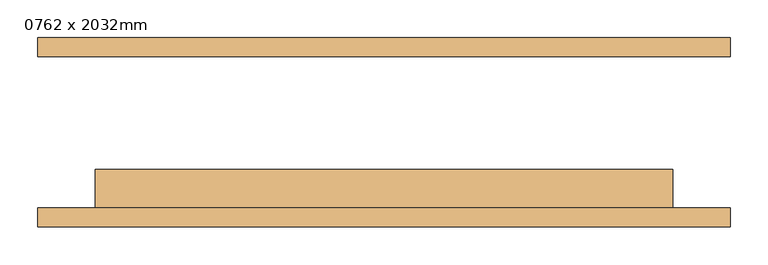
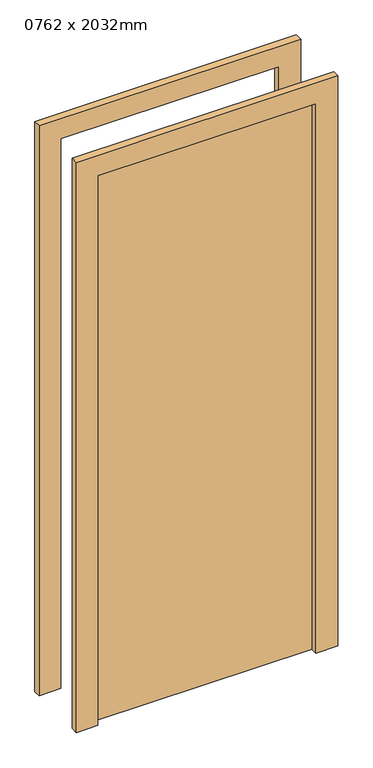
"""IFC4 building model written with IfcOpenShell, lengths in millimetres: door geometry, M_Folha única : 0762 x 2032mm."""

import ifcopenshell
import ifcopenshell.guid

model = None  # the IFC model being written
_history = None  # IfcOwnerHistory: only IFC2X3 demands one
_inside = {}  # id of a spatial element -> (the spatial element, [elements in it])
_under = {}  # id of a project, library or spatial element -> (it, [spatial elements below it])
_declared = {}  # id of a project -> (the project, [libraries it declares])
_typed = {}  # id of a type object -> (the type object, [elements of that type])
_made_of = {}  # id of a material, layer set ... -> (it, [elements and type objects made of it])


def new_model(schema):
    """Start an empty IFC model of exactly this schema.

    Asked for "IFC4X3", IfcOpenShell would pick the latest addendum, in which some entities
    have other attributes; the version numbers below select the first issue.
    IFC2X3 requires an IfcOwnerHistory on every rooted entity: one is made here for all.
    """
    global model, _history
    if schema == "IFC4X3":
        model = ifcopenshell.file(schema_version=(4, 3, 0, 0))
    else:
        model = ifcopenshell.file(schema=schema)
    _inside.clear()
    _under.clear()
    _declared.clear()
    _typed.clear()
    _made_of.clear()
    _history = None
    if model.schema == "IFC2X3":
        org = make("IfcOrganization", Name="unknown")
        user = make(
            "IfcPersonAndOrganization",
            ThePerson=make("IfcPerson", FamilyName="unknown"),
            TheOrganization=org,
        )
        app = make(
            "IfcApplication",
            ApplicationDeveloper=org,
            Version="unknown",
            ApplicationFullName="unknown",
            ApplicationIdentifier="unknown",
        )
        _history = make(
            "IfcOwnerHistory",
            OwningUser=user,
            OwningApplication=app,
            ChangeAction="ADDED",
            CreationDate=0,
        )
    return model


def make(cls, **values):
    """One entity of the class cls with the attributes given. An attribute that is None is left unset."""
    return model.create_entity(
        cls, **{name: value for name, value in values.items() if value is not None}
    )


def rooted(cls, **values):
    """An entity with a GlobalId (a new one), such as an element, a storey or a relation."""
    return make(cls, GlobalId=ifcopenshell.guid.new(), OwnerHistory=_history, **values)


def si_unit(unit_type, name, prefix=None):
    """IfcSIUnit, for example si_unit("LENGTHUNIT", "METRE", prefix="MILLI")."""
    return make("IfcSIUnit", UnitType=unit_type, Prefix=prefix, Name=name)


def assignment(units):
    """IfcUnitAssignment: the units of a project."""
    return None if units is None else make("IfcUnitAssignment", Units=units)


def point(xyz):
    """IfcCartesianPoint."""
    return None if xyz is None else make("IfcCartesianPoint", Coordinates=xyz)


def direction(xyz):
    """IfcDirection."""
    return None if xyz is None else make("IfcDirection", DirectionRatios=xyz)


def frame(location, z_axis=None, x_axis=None):
    """IfcAxis2Placement3D, a coordinate frame: its origin and axes. An axis left out is left unset."""
    return make(
        "IfcAxis2Placement3D",
        Location=point(location),
        Axis=direction(z_axis),
        RefDirection=direction(x_axis),
    )


def origin():
    """The frame at (0, 0, 0) with its axes left unset."""
    return frame((0.0, 0.0, 0.0))


def origin_with_axes():
    """The frame at (0, 0, 0) with the z axis (0, 0, 1) and the x axis (1, 0, 0) written out."""
    return frame((0.0, 0.0, 0.0), z_axis=(0.0, 0.0, 1.0), x_axis=(1.0, 0.0, 0.0))


def place(relative_to, where):
    """IfcLocalPlacement: puts the frame where relative to a parent placement (None: the world)."""
    return make(
        "IfcLocalPlacement", PlacementRelTo=relative_to, RelativePlacement=where
    )


def context(
    kind, dimensions, precision=None, world=None, true_north=None, identifier=None
):
    """IfcGeometricRepresentationContext, for example the 3D "Model" context."""
    return make(
        "IfcGeometricRepresentationContext",
        ContextIdentifier=identifier,
        ContextType=kind,
        CoordinateSpaceDimension=dimensions,
        Precision=precision,
        WorldCoordinateSystem=world,
        TrueNorth=true_north,
    )


def project(units=None, contexts=None):
    """IfcProject with its units and contexts."""
    return rooted(
        "IfcProject",
        Name="project",
        RepresentationContexts=contexts,
        UnitsInContext=assignment(units),
    )


def spatial(cls, under=None, at=None, **own):
    """A site, building, storey or space (cls), placed at a placement, below another one or the project."""
    s = rooted(cls, ObjectPlacement=at, **own)
    if under is not None:
        _under.setdefault(under.id(), (under, []))[1].append(s)
    return s


def polyline(points):
    """IfcPolyline through the points."""
    return make("IfcPolyline", Points=[point(p) for p in points])


def outline(outer, holes=None, kind="AREA"):
    """IfcArbitraryClosedProfileDef: a profile drawn as a closed curve; with holes, ...WithVoids."""
    if holes is None:
        return make("IfcArbitraryClosedProfileDef", ProfileType=kind, OuterCurve=outer)
    return make(
        "IfcArbitraryProfileDefWithVoids",
        ProfileType=kind,
        OuterCurve=outer,
        InnerCurves=holes,
    )


def extrude(swept, where, along, depth):
    """IfcExtrudedAreaSolid: the profile swept, set in the frame where, extruded along a direction by depth."""
    return make(
        "IfcExtrudedAreaSolid",
        SweptArea=swept,
        Position=where,
        ExtrudedDirection=direction(along),
        Depth=depth,
    )


def shape(context_of_items, identifier, shape_type, items):
    """IfcShapeRepresentation: the items that make up one representation, for example the "Body"."""
    return make(
        "IfcShapeRepresentation",
        ContextOfItems=context_of_items,
        RepresentationIdentifier=identifier,
        RepresentationType=shape_type,
        Items=items,
    )


def source(mapping_origin, context_of_items, identifier, shape_type, items):
    """IfcRepresentationMap: a shape defined once, which mapped items show again and again."""
    return make(
        "IfcRepresentationMap",
        MappingOrigin=mapping_origin,
        MappedRepresentation=shape(context_of_items, identifier, shape_type, items),
    )


def transform(
    local_origin,
    x_axis=None,
    y_axis=None,
    z_axis=None,
    scale=None,
    scale2=None,
    scale3=None,
    uniform=True,
):
    """IfcCartesianTransformationOperator3D, or its non-uniform kind. x_axis, y_axis, z_axis: its Axis1, 2, 3."""
    if uniform:
        return make(
            "IfcCartesianTransformationOperator3D",
            Axis1=direction(x_axis),
            Axis2=direction(y_axis),
            LocalOrigin=point(local_origin),
            Scale=scale,
            Axis3=direction(z_axis),
        )
    return make(
        "IfcCartesianTransformationOperator3DnonUniform",
        Axis1=direction(x_axis),
        Axis2=direction(y_axis),
        LocalOrigin=point(local_origin),
        Scale=scale,
        Axis3=direction(z_axis),
        Scale2=scale2,
        Scale3=scale3,
    )


def mapped(mapping_source, mapping_target):
    """IfcMappedItem: shows the shape of a source again, moved by a transform."""
    return make(
        "IfcMappedItem", MappingSource=mapping_source, MappingTarget=mapping_target
    )


def made_of(thing, what):
    """Note that an element or type object is made of a material, layer set ...; save() writes the relation."""
    if what is not None:
        _made_of.setdefault(what.id(), (what, []))[1].append(thing)
    return thing


def element(
    cls,
    number,
    at=None,
    inside=None,
    cuts=None,
    type_object=None,
    material=None,
    context=None,
    identifier="Body",
    shape_type=None,
    held_by="IfcProductDefinitionShape",
    body=None,
    shapes=None,
    **own,
):
    """One element of the class cls, such as IfcWall. Its Tag is "e" and its number.

    at: its placement. inside: the storey or other place that contains it. cuts: it is an
    opening in that element (IfcRelVoidsElement). A single representation is given by context,
    identifier, shape_type and body (its items); several are given by shapes. held_by: the class
    of the entity that holds the representations. save() writes the other relations.
    """
    e = rooted(cls, Tag="e%d" % number, ObjectPlacement=at, **own)
    if body is not None:
        shapes = [shape(context, identifier, shape_type, body)]
    if shapes is not None:
        e.Representation = make(held_by, Representations=shapes)
    if inside is not None:
        _inside.setdefault(inside.id(), (inside, []))[1].append(e)
    if cuts is not None:
        rooted(
            "IfcRelVoidsElement", RelatingBuildingElement=cuts, RelatedOpeningElement=e
        )
    if type_object is not None:
        _typed.setdefault(type_object.id(), (type_object, []))[1].append(e)
    return made_of(e, material)


def aggregate(whole, parts):
    """IfcRelAggregates: a whole, such as a stair, and the parts it consists of."""
    return rooted("IfcRelAggregates", RelatingObject=whole, RelatedObjects=parts)


def save(model, path):
    """Write the relations noted so far, then the file.

    IfcRelAggregates (storeys below a building ...), IfcRelContainedInSpatialStructure (elements
    in a storey), IfcRelDefinesByType, IfcRelAssociatesMaterial and IfcRelDeclares: one each for
    every whole, place, type object, material and project.
    """
    for whole, parts in _under.values():
        aggregate(whole, parts)
    for where, things in _inside.values():
        rooted(
            "IfcRelContainedInSpatialStructure",
            RelatedElements=things,
            RelatingStructure=where,
        )
    for kind, things in _typed.values():
        rooted("IfcRelDefinesByType", RelatedObjects=things, RelatingType=kind)
    for what, things in _made_of.values():
        rooted("IfcRelAssociatesMaterial", RelatedObjects=things, RelatingMaterial=what)
    for by, libraries in _declared.values():
        rooted("IfcRelDeclares", RelatingContext=by, RelatedDefinitions=libraries)
    model.write(path)


def door_0762_x_2032mm_7341a4fb(model_context):
    return source(origin(), model_context, "Body", "SweptSolid", [
        extrude(outline(polyline([(2108.0, -457.0), (0.0, -457.0), (0.0, -381.0), (2032.0, -381.0), (2032.0, 381.0), (0.0, 381.0), (0.0, 457.0), (2108.0, 457.0), (2108.0, -457.0)])), frame((0.0, -125.0, 0.0), z_axis=(0.0, 1.0, 0.0), x_axis=(0.0, 0.0, 1.0)), (0.0, 0.0, 1.0), 25.0),
        extrude(outline(polyline([(2108.0, 457.0), (2108.0, -457.0), (0.0, -457.0), (0.0, -381.0), (2032.0, -381.0), (2032.0, 381.0), (0.0, 381.0), (0.0, 457.0), (2108.0, 457.0)])), frame((0.0, 100.0, 0.0), z_axis=(0.0, 1.0, 0.0), x_axis=(0.0, 0.0, 1.0)), (0.0, 0.0, 1.0), 25.0),
        extrude(outline(polyline([(381.0, -49.0), (381.0, -100.0), (-381.0, -100.0), (-381.0, -49.0), (381.0, -49.0)])), origin_with_axes(), (0.0, 0.0, 1.0), 2032.0),
    ])


if __name__ == "__main__":
    model = new_model("IFC4")
    model_context = context("Model", 3, world=origin())
    ifc_project = project(units=[si_unit("LENGTHUNIT", "METRE", prefix="MILLI")], contexts=[model_context])
    site = spatial("IfcSite", under=ifc_project)
    building = spatial("IfcBuilding", under=site)
    placement = place(None, origin())
    door_0762_x_2032mm_shape = door_0762_x_2032mm_7341a4fb(model_context)
    element("IfcDoor", 1, ObjectType="M_Folha única : 0762 x 2032mm", at=placement, inside=building, context=model_context, shape_type="MappedRepresentation", body=[
        mapped(door_0762_x_2032mm_shape, transform((0.0, 0.0, 0.0), x_axis=(1.0, 0.0, 0.0), y_axis=(0.0, 1.0, 0.0), z_axis=(0.0, 0.0, 1.0))),
    ])
    save(model, "model.ifc")

# Revit data of these elements
# Type "M_Folha única : 0762 x 2032mm"
#   Type Mark = "28"
#   Construction Type Id = "MDOOR"
#   Analytic Construction = "Metal"
#   Thickness = 0.051 m
#   Thermal Resistance (R) = 0.270117 (m²·K)/W
#   Heat Transfer Coefficient (U) = 3.7021 W/(m²·K)
#   Height = 2.032 m
#   Projeção da apara externa = 0.025 m
#   Projeção da apara interna = 0.025 m
#   Largura da apara = 0.076 m
#   Width = 0.762 m
#   semi_oca = no
#   Define Thermal Properties by = 1
#   Material da porta = Porta - Painel
#   Material da moldura = Porta - Batente
#   Visual Light Transmittance = 0
#   Solar Heat Gain Coefficient = 0
#   Function = (empty or 0)
#   Wall Closure = (empty or 0)
# Element 1 (IfcDoor, "M_Folha única : 0762 x 2032mm")
#   Materials on its faces: "Porta - Batente", "Porta - Painel"
# Materials
#   "Porta - Painel": class "Madeira", colour RGB 210 159 95, transparency 0, Cost = 0
#   "Porta - Batente": class "Diversos", colour RGB 118 70 51, transparency 0, Cost = 0
